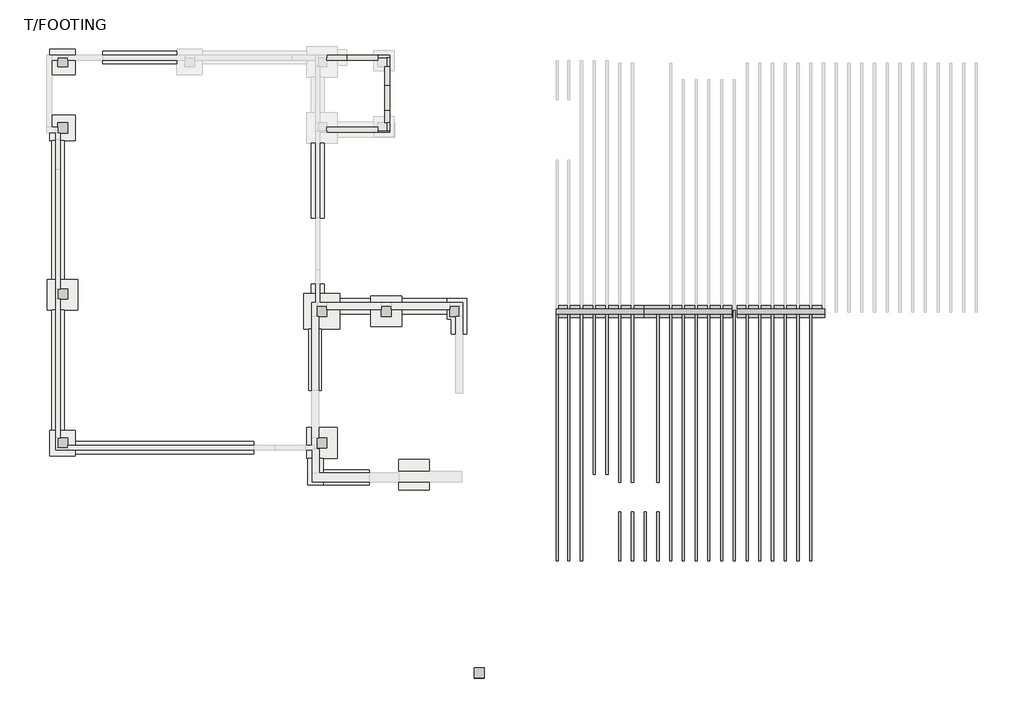
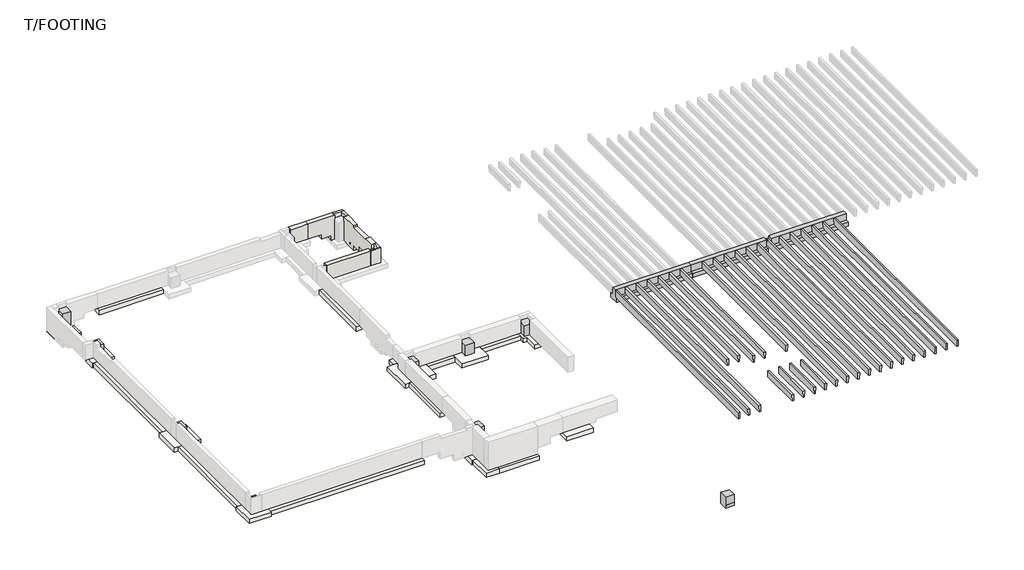
# One storey, part 2 of 3: 27 beams, 11 footings, 9 columns, 9 slabs, 8 walls.
# Revit data of these elements (continued)
# Type "Precast-Cone Shaped Beam : DOUBLE_T"
#   Top Width = 0' - 5"
#   Tie Rod Weight [instance default] = 30
#   Tie Rod W [instance default] = 0.0660938 kip
#   Single Rebar Weight [instance default] = 50
#   Single Rebar W [instance default] = 0.110156 kip
#   Rebar Grids Weight [instance default] = 100
#   Rebar Grids W [instance default] = 0.220313 kip
#   Depth = 1' - 6"
#   Bottom Width = 0' - 4"
#   Length [instance default] = 5' - 0"
#   Structural Material [instance default] = Concrete, Precast
#   Assembly Code = ""
# Type "Precast-Inverted Tee : 20+12X28"
#   Assembly Code = "B10"
#   Seat = 0' - 8"
#   Length [instance default] = 5' - 0"
#   b = 2' - 4"
#   h = 2' - 8"
#   h1 = 1' - 8"
#   Structural Material [instance default] = Concrete - Precast Concrete - Normal Weight Concrete - 5 ksi
# Type "Concrete-Square-Column : PIER 24\"x24\""
#   Assembly Code = "B10"
#   b = 2' - 0"
#   Structural Material [instance default] = Concrete, Cast-in-Place gray
# Type "F4"
#   Assembly Code = "A1010110"
# Type "WF_30IN"
#   Assembly Code = "A1010110"
# Type "12\" Foundation SLAB"
#   Layers, outside or top first: 1' - 0" "Concrete, Cast-in-Place gray" (function 1)
# Type "Spread Footing - Rectangular : F5"
#   Trans Top Reinf = ""
#   Trans Bot Reinf = "6#6"
#   Long Top Reinf = ""
#   Long Bot Reinf = "6#6"
#   Foundation Mark = "F5"
#   Assembly Code = "A1010100"
#   Width = 5' - 0"
#   Length = 5' - 0"
#   Foundation Thickness = 1' - 0"
#   Thickness = 1' - 0"
#   Structural Material [instance default] = Concrete - Cast-in-Place Concrete
# Type "Spread Footing - Rectangular : F6"
#   Trans Top Reinf = ""
#   Trans Bot Reinf = "7#6"
#   Long Top Reinf = ""
#   Long Bot Reinf = "7#6"
#   Foundation Mark = "F6"
#   Assembly Code = "A1010100"
#   Width = 6' - 0"
#   Length = 6' - 0"
#   Foundation Thickness = 1' - 0"
#   Thickness = 1' - 0"
#   Structural Material [instance default] = Concrete - Cast-in-Place Concrete
# Type "Spread Footing - Rectangular : F7"
#   Trans Top Reinf = ""
#   Trans Bot Reinf = "8#6"
#   Long Top Reinf = ""
#   Long Bot Reinf = "8#6"
#   Foundation Mark = "F7"
#   Assembly Code = "A1010100"
#   Width = 7' - 0"
#   Length = 7' - 0"
#   Foundation Thickness = 1' - 0"
#   Thickness = 1' - 0"
#   Structural Material [instance default] = Concrete - Cast-in-Place Concrete
# Type "12\" CONCRETE WALL"
#   Assembly Code = "B2010158"
#   Layers, outside or top first: 1' - 0" "Concrete, Cast-in-Place gray" (function 1)
# Type "2\" CONCRETE WALL"
#   Assembly Code = "B2010158"
#   Layers, outside or top first: 0' - 2" "Concrete, Cast-in-Place gray" (function 1)
# Type "6\" CONCRETE WALL"
#   Assembly Code = "B2010158"
#   Layers, outside or top first: 0' - 6" "Concrete, Cast-in-Place gray" (function 1)
# Elements 1, 2, 3, 4, 5, 6, 7, 8, 9, 10, 11, 12, 13, 14, 15 (IfcBeam, "Precast-Cone Shaped Beam : DOUBLE_T")
#   Comments = ""
#   Tie Rod Weight = 30
#   Tie Rod W = 0.0660938 kip
#   Single Rebar Weight = 50
#   Single Rebar W = 0.110156 kip
#   Rebar Grids Weight = 100
#   Rebar Grids W = 0.220313 kip
#   Length = 49' - 6"
#   Structural Material = Concrete - Precast Concrete - Normal Weight Concrete - 5 ksi
#   Phase Created = New Construction
#   Materials on its faces: "Concrete - Precast Concrete - Normal Weight Concrete - 5 ksi"
# Elements 16, 17, 18 (IfcBeam, "Precast-Cone Shaped Beam : DOUBLE_T")
#   Comments = ""
#   Tie Rod Weight = 30
#   Tie Rod W = 0.0660938 kip
#   Single Rebar Weight = 50
#   Single Rebar W = 0.110156 kip
#   Rebar Grids Weight = 100
#   Rebar Grids W = 0.220313 kip
#   Length = 33' - 1 3/16"
#   Structural Material = Concrete - Precast Concrete - Normal Weight Concrete - 5 ksi
#   Phase Created = New Construction
#   Materials on its faces: "Concrete - Precast Concrete - Normal Weight Concrete - 5 ksi"
# Elements 19, 20, 21, 22 (IfcBeam, "Precast-Cone Shaped Beam : DOUBLE_T")
#   Comments = ""
#   Tie Rod Weight = 30
#   Tie Rod W = 0.0660938 kip
#   Single Rebar Weight = 50
#   Single Rebar W = 0.110156 kip
#   Rebar Grids Weight = 100
#   Rebar Grids W = 0.220313 kip
#   Length = 9' - 7 3/16"
#   Structural Material = Concrete - Precast Concrete - Normal Weight Concrete - 5 ksi
#   Phase Created = New Construction
#   Materials on its faces: "Concrete - Precast Concrete - Normal Weight Concrete - 5 ksi"
# Elements 23, 24 (IfcBeam, "Precast-Cone Shaped Beam : DOUBLE_T")
#   Comments = ""
#   Tie Rod Weight = 30
#   Tie Rod W = 0.0660938 kip
#   Single Rebar Weight = 50
#   Single Rebar W = 0.110156 kip
#   Rebar Grids Weight = 100
#   Rebar Grids W = 0.220313 kip
#   Length = 31' - 7"
#   Structural Material = Concrete - Precast Concrete - Normal Weight Concrete - 5 ksi
#   Phase Created = New Construction
#   Materials on its faces: "Concrete - Precast Concrete - Normal Weight Concrete - 5 ksi"
# Element 25 (IfcBeam, "Precast-Inverted Tee : 20+12X28")
#   Length = 17' - 5.84473"
#   Structural Material = Concrete - Precast Concrete - Normal Weight Concrete - 5 ksi
#   Phase Created = Existing
#   Materials on its faces: "Concrete - Precast Concrete - Normal Weight Concrete - 5 ksi"
# Element 26 (IfcBeam, "Precast-Inverted Tee : 20+12X28")
#   Length = 17' - 3"
#   Structural Material = Concrete - Precast Concrete - Normal Weight Concrete - 5 ksi
#   Phase Created = Existing
#   Materials on its faces: "Concrete - Precast Concrete - Normal Weight Concrete - 5 ksi"
# Element 27 (IfcBeam, "Precast-Inverted Tee : 20+12X28")
#   Length = 17' - 6"
#   Structural Material = Concrete - Precast Concrete - Normal Weight Concrete - 5 ksi
#   Phase Created = Existing
#   Materials on its faces: "Concrete - Precast Concrete - Normal Weight Concrete - 5 ksi"
# Elements 28, 29, 30, 31, 32, 33, 34, 35, 36 (IfcColumn, "Concrete-Square-Column : PIER 24\"x24\"")
#   Comments = ""
#   Structural Material = Concrete, Cast-in-Place gray
#   Phase Created = New Construction
#   Materials on its faces: "Concrete, Cast-in-Place gray"
# Element 37 (IfcFooting, "F4")
#   Comments = ""
#   Phase Created = New Construction
#   Materials on its faces: "Concrete - Cast-in-Place Concrete"
# Elements 38, 39, 40 (IfcFooting, "F4")
#   Phase Created = New Construction
#   Materials on its faces: "Concrete - Cast-in-Place Concrete"
# Elements 41, 43, 44, 45, 46, 47 (IfcFooting, "WF_30IN")
#   Phase Created = New Construction
#   Materials on its faces: "Default Floor"
# Element 42 (IfcFooting, "WF_30IN")
#   Comments = ""
#   Phase Created = New Construction
#   Materials on its faces: "Default Floor"
# Element 48 (IfcSlab, "12\" Foundation SLAB")
#   Comments = ""
#   Height Offset From Level = 0' - 0"
#   built-in parameter 1001954 = 1
#   Phase Created = New Construction
#   Materials on its faces: "Concrete, Cast-in-Place gray"
# Element 49 (IfcSlab, "Spread Footing - Rectangular : F5")
#   Structural Material = Concrete, Cast-in-Place gray
#   Phase Created = New Construction
#   Materials on its faces: "Concrete, Cast-in-Place gray"
# Elements 50, 51 (IfcSlab, "Spread Footing - Rectangular : F5")
#   Comments = ""
#   Structural Material = Concrete, Cast-in-Place gray
#   Phase Created = New Construction
#   Materials on its faces: "Concrete, Cast-in-Place gray"
# Elements 52, 53, 54, 55 (IfcSlab, "Spread Footing - Rectangular : F6")
#   Comments = ""
#   Structural Material = Concrete, Cast-in-Place gray
#   Phase Created = New Construction
#   Materials on its faces: "Concrete, Cast-in-Place gray"
# Element 56 (IfcSlab, "Spread Footing - Rectangular : F7")
#   Comments = ""
#   Structural Material = Concrete, Cast-in-Place gray
#   Phase Created = New Construction
#   Materials on its faces: "Concrete, Cast-in-Place gray"
# Elements 57, 58, 59, 60 (IfcWall, "12\" CONCRETE WALL")
#   Comments = ""
#   Top Offset = 0' - 0"
#   Base Offset = 0' - 0"
#   wall height = 3' - 7"
#   Phase Created = New Construction
#   Base Constraint = T/FOOTING
#   Top Constraint = MAIN LEVEL FLOOR PLAN
#   Materials on its faces: "Concrete, Cast-in-Place gray"
# Element 61 (IfcWall, "2\" CONCRETE WALL")
#   Comments = ""
#   Top Offset = 0' - 0"
#   Base Offset = 0' - 0"
#   wall height = 3' - 7"
#   Phase Created = New Construction
#   Base Constraint = T/FOOTING
#   Top Constraint = MAIN LEVEL FLOOR PLAN
#   Materials on its faces: "Concrete, Cast-in-Place gray"
# Elements 62, 63 (IfcWall, "6\" CONCRETE WALL")
#   Comments = ""
#   built-in parameter 1001111 = -2' - 2"
#   Top Offset = 0' - 0"
#   Base Offset = -2' - 2"
#   wall height = 5' - 9"
#   Phase Created = New Construction
#   Base Constraint = T/FOOTING
#   Top Constraint = MAIN LEVEL FLOOR PLAN
#   Materials on its faces: "Concrete, Cast-in-Place gray"
# Element 64 (IfcWall, "6\" CONCRETE WALL")
#   Comments = ""
#   Top Offset = 0' - 0"
#   Base Offset = 0' - 0"
#   wall height = 3' - 7"
#   Phase Created = New Construction
#   Base Constraint = T/FOOTING
#   Top Constraint = MAIN LEVEL FLOOR PLAN
#   Materials on its faces: "Concrete, Cast-in-Place gray"
# Materials
#   "Concrete, Precast": class "Concrete", colour RGB 198 187 187, transparency 0, Description = "Precast concrete", Cost = 0
#   "Concrete - Precast Concrete - Normal Weight Concrete - 5 ksi": class "Concrete", colour RGB 198 187 187, transparency 0, Cost = 0
#   "Concrete, Cast-in-Place gray": class "Concrete", colour RGB 192 192 192, transparency 0, Description = "Cast-in-place concrete", Cost = 0
#   "Concrete - Cast-in-Place Concrete": class "Concrete", colour RGB 192 192 192, transparency 0, Description = "Concrete", Cost = 0
#   "Default Floor": class "Miscellaneous", colour RGB 128 128 128, transparency 0, Cost = 0
